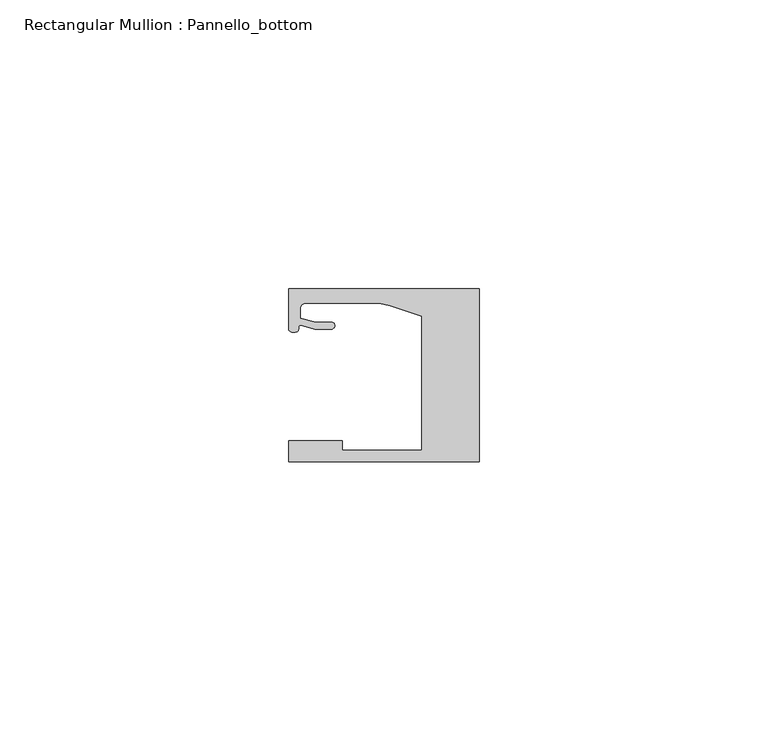
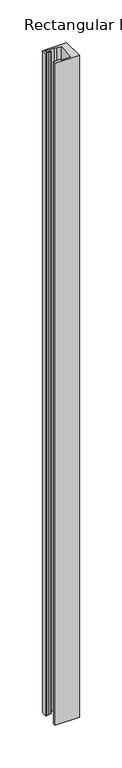
"""IFC4 building model written with IfcOpenShell, lengths in millimetres: member geometry, Rectangular Mullion : Pannello_bottom."""

from ifc_helpers import new_model, si_unit, frame, origin, place, context, project, spatial, polyline, circle_curve, source, transform, mapped, element, save
from ifc_brep_helpers import plane_surface, cylinder_surface, revolved_surface, extruded_surface, spline_curve, advanced_brep


def rectangular_mullion_pannello_bottom_0ebbe626(model_context):
    return source(origin(), model_context, "Body", "AdvancedBrep", [
        advanced_brep(
        [(-33.0, -15.0, 0.0), (0.0, -15.0, 0.0), (0.0, 15.0, 0.0), (-33.0000135, 15.0, 0.0), (-33.0000135, 8.0000472, 0.0), (-30.9223017, 8.6490241, 0.0), (-28.4999305, 7.9999523, 0.0), (-25.59998, 7.9999523, 0.0), (-25.59998, 9.1999523, 0.0), (-28.3419477, 9.1999523, 0.0), (-31.0, 9.9121746, 0.0), (-31.0, 11.4999419, 0.0), (-30.0000002, 12.4999419, 0.0), (-18.5493024, 12.4999438, 0.0), (-15.4591336, 12.0105099, 0.0), (-9.9999723, 10.2367227, 0.0), (-9.9999723, -13.0000004, 0.0), (-23.700041, -13.0000004, 0.0), (-23.700041, -11.3000004, 0.0), (-33.0, -11.3000004, 0.0), (-33.0, -15.0, -950.0), (-33.0, -11.3000004, -950.0), (-23.700041, -11.3000004, -950.0), (-23.700041, -13.0000004, -950.0), (-9.9999723, -13.0000004, -950.0), (-9.9999723, 10.2367227, -950.0), (-15.4591336, 12.0105099, -950.0), (-18.5493024, 12.4999438, -950.0), (-30.0000002, 12.4999419, -950.0), (-31.0, 11.4999419, -950.0), (-31.0, 9.9121746, -950.0), (-28.3419477, 9.1999523, -950.0), (-25.59998, 9.1999523, -950.0), (-25.59998, 7.9999523, -950.0), (-28.4999305, 7.9999523, -950.0), (-30.9223017, 8.6490241, -950.0), (-33.0000135, 8.0000472, -950.0), (-33.0000135, 15.0, -950.0), (0.0, 15.0, -950.0), (0.0, -15.0, -950.0)],
        [
            (0, 1),
            (1, 2),
            (2, 3),
            (3, 4),
            (4, 5, spline_curve(3, [(-33.0000135, 8.0000472, 0.0), (-33.0000135, 7.457047519, 0.0), (-32.262327879, 7.456527435, 0.0), (-31.357433266, 7.563996614, 0.0), (-31.305645054, 7.690065204, 0.0), (-31.298563602, 8.366228555, 0.0), (-31.312054066, 8.717747958, 0.0), (-30.9223017, 8.6490241, 0.0)], [4, 2, 2, 4], [0.0, 0.0027053965905959043, 0.0058611956533709, 0.007702013405570312])),
            (5, 6),
            (6, 7),
            (7, 8, circle_curve(frame((-25.59998, 8.5999523, 0.0), z_axis=(0.0, 0.0, 1.0), x_axis=(0.0, 1.0, 0.0)), 0.6)),
            (8, 9),
            (9, 10),
            (10, 11),
            (11, 12, circle_curve(frame((-30.0, 11.4999419, 0.0), z_axis=(0.0, 0.0, -1.0), x_axis=(0.0, 1.0, 0.0)), 1.0)),
            (12, 13),
            (13, 14, circle_curve(frame((-18.5493007, 2.4999438, 0.0), z_axis=(0.0, 0.0, -1.0), x_axis=(0.0, 1.0, 0.0)), 10.0)),
            (14, 15),
            (15, 16),
            (16, 17),
            (17, 18),
            (18, 19),
            (19, 0),
            (20, 21),
            (21, 22),
            (22, 23),
            (23, 24),
            (24, 25),
            (25, 26),
            (26, 27, circle_curve(frame((-18.5493007, 2.4999438, -950.0), z_axis=(0.0, 0.0, 1.0), x_axis=(0.0, 1.0, 0.0)), 10.0)),
            (27, 28),
            (28, 29, circle_curve(frame((-30.0, 11.4999419, -950.0), z_axis=(0.0, 0.0, 1.0), x_axis=(0.0, 1.0, 0.0)), 1.0)),
            (29, 30),
            (30, 31),
            (31, 32),
            (32, 33, circle_curve(frame((-25.59998, 8.5999523, -950.0), z_axis=(0.0, 0.0, -1.0), x_axis=(0.0, 1.0, 0.0)), 0.6)),
            (33, 34),
            (34, 35),
            (35, 36, spline_curve(3, [(-30.9223017, 8.6490241, -950.0), (-31.312054066, 8.717747958, -950.0), (-31.298563602, 8.366228555, -950.0), (-31.305645054, 7.690065204, -950.0), (-31.357433266, 7.563996614, -950.0), (-32.262327879, 7.456527435, -950.0), (-33.0000135, 7.457047519, -950.0), (-33.0000135, 8.0000472, -950.0)], [4, 2, 2, 4], [0.0, 0.001840817752199412, 0.004996616814974408, 0.007702013405570312])),
            (36, 37),
            (37, 38),
            (38, 39),
            (39, 20),
            (0, 20),
            (39, 1),
            (38, 2),
            (37, 3),
            (36, 4),
            (35, 5),
            (34, 6),
            (33, 7),
            (32, 8),
            (31, 9),
            (30, 10),
            (29, 11),
            (28, 12),
            (27, 13),
            (26, 14),
            (25, 15),
            (24, 16),
            (23, 17),
            (22, 18),
            (21, 19),
        ],
        [
            plane_surface(frame((0.0, -36.2491502, 0.0), z_axis=(0.0, 0.0, 1.0), x_axis=(-1.0, 0.0, 0.0))),
            plane_surface(frame((0.0, -36.2491502, -950.0), z_axis=(0.0, 0.0, -1.0), x_axis=(-1.0, 0.0, 0.0))),
            plane_surface(frame((-33.0, -15.0, 0.0), z_axis=(0.0, -1.0, 0.0), x_axis=(0.0, 0.0, -1.0))),
            plane_surface(frame((0.0, -15.0, 0.0), z_axis=(1.0, 0.0, 0.0), x_axis=(0.0, 0.0, -1.0))),
            plane_surface(frame((0.0, 15.0, 0.0), z_axis=(0.0, 1.0, 0.0), x_axis=(0.0, 0.0, -1.0))),
            plane_surface(frame((-33.0000135, 15.0, 0.0), z_axis=(-1.0, 0.0, 0.0), x_axis=(0.0, 0.0, -1.0))),
            extruded_surface(spline_curve(3, [(-33.0000135, 8.0000472, -950.0), (-33.0000135, 7.457047519, -950.0), (-32.262327879, 7.456527435, -950.0), (-31.357433266, 7.563996614, -950.0), (-31.305645054, 7.690065204, -950.0), (-31.298563602, 8.366228555, -950.0), (-31.312054066, 8.717747958, -950.0), (-30.9223017, 8.6490241, -950.0)], [4, 2, 2, 4], [0.0, 0.0027053965905959043, 0.0058611956533709, 0.007702013405570312]), (0.0, 0.0, 950.0), 950.0),
            plane_surface(frame((-30.9223017, 8.6490241, 0.0), z_axis=(-0.25881883200192934, -0.9659258833891746, 0.0), x_axis=(0.0, 0.0, -1.0))),
            plane_surface(frame((-28.4999305, 7.9999523, 0.0), z_axis=(0.0, -1.0, 0.0), x_axis=(0.0, 0.0, -1.0))),
            cylinder_surface(frame((-25.59998, 8.5999523, 0.0), z_axis=(0.0, 0.0, 1.0), x_axis=(0.0, 1.0, 0.0)), 0.6),
            plane_surface(frame((-25.59998, 9.1999523, 0.0), z_axis=(0.0, 1.0, 0.0), x_axis=(0.0, 0.0, -1.0))),
            plane_surface(frame((-28.3419477, 9.1999523, 0.0), z_axis=(0.25881883204288636, 0.9659258833782002, 0.0), x_axis=(0.0, 0.0, -1.0))),
            plane_surface(frame((-31.0, 9.9121746, 0.0), z_axis=(1.0, 0.0, 0.0), x_axis=(0.0, 0.0, -1.0))),
            revolved_surface(polyline([(-30.0, 12.4999419, -950.0), (-30.0, 12.4999419, 0.0)]), (-30.0, 11.4999419, 0.0), (0.0, 0.0, -1.0)),
            plane_surface(frame((-30.0000002, 12.4999419, 0.0), z_axis=(1.6923026533778639e-07, -0.9999999999999858, 0.0), x_axis=(0.0, 0.0, -1.0))),
            revolved_surface(polyline([(-18.5493007, 12.4999438, -950.0), (-18.5493007, 12.4999438, 0.0)]), (-18.5493007, 2.4999438, 0.0), (0.0, 0.0, -1.0)),
            plane_surface(frame((-15.4591336, 12.0105099, 0.0), z_axis=(-0.30901670911956314, -0.9510566089801992, 0.0), x_axis=(0.0, 0.0, -1.0))),
            plane_surface(frame((-9.9999723, 10.2367227, 0.0), z_axis=(-1.0, 0.0, 0.0), x_axis=(0.0, 0.0, -1.0))),
            plane_surface(frame((-9.9999723, -13.0000004, 0.0), z_axis=(0.0, 1.0, 0.0), x_axis=(0.0, 0.0, -1.0))),
            plane_surface(frame((-23.700041, -13.0000004, 0.0), z_axis=(1.0, 0.0, 0.0), x_axis=(0.0, 0.0, -1.0))),
            plane_surface(frame((-23.700041, -11.3000004, 0.0), z_axis=(0.0, 1.0, 0.0), x_axis=(0.0, 0.0, -1.0))),
            plane_surface(frame((-33.0, -11.3000004, 0.0), z_axis=(-1.0, 0.0, 0.0), x_axis=(0.0, 0.0, -1.0))),
        ],
        [
            (0, [[1, 2, 3, 4, 5, 6, 7, 8, 9, 10, 11, 12, 13, 14, 15, 16, 17, 18, 19, 20]]),
            (1, [[21, 22, 23, 24, 25, 26, 27, 28, 29, 30, 31, 32, 33, 34, 35, 36, 37, 38, 39, 40]]),
            (2, [[-1, 41, -40, 42]]),
            (3, [[-2, -42, -39, 43]]),
            (4, [[-3, -43, -38, 44]]),
            (5, [[-4, -44, -37, 45]]),
            (6, [[-5, -45, -36, 46]]),
            (7, [[-6, -46, -35, 47]]),
            (8, [[-7, -47, -34, 48]]),
            (9, [[-8, -48, -33, 49]]),
            (10, [[-9, -49, -32, 50]]),
            (11, [[-10, -50, -31, 51]]),
            (12, [[-11, -51, -30, 52]]),
            (13, [[-12, -52, -29, 53]]),
            (14, [[-13, -53, -28, 54]]),
            (15, [[-14, -54, -27, 55]]),
            (16, [[-15, -55, -26, 56]]),
            (17, [[-16, -56, -25, 57]]),
            (18, [[-17, -57, -24, 58]]),
            (19, [[-18, -58, -23, 59]]),
            (20, [[-19, -59, -22, 60]]),
            (21, [[-20, -60, -21, -41]]),
        ],
    ),
    ])


if __name__ == "__main__":
    model = new_model("IFC4")
    model_context = context("Model", 3, world=origin())
    ifc_project = project(units=[si_unit("LENGTHUNIT", "METRE", prefix="MILLI")], contexts=[model_context])
    site = spatial("IfcSite", under=ifc_project)
    building = spatial("IfcBuilding", under=site)
    placement = place(None, origin())
    rectangular_mullion_pannello_bottom_shape = rectangular_mullion_pannello_bottom_0ebbe626(model_context)
    element("IfcMember", 1, ObjectType="Rectangular Mullion : Pannello_bottom", at=placement, inside=building, context=model_context, shape_type="MappedRepresentation", body=[
        mapped(rectangular_mullion_pannello_bottom_shape, transform((0.0, 0.0, 0.0), x_axis=(1.0, 0.0, 0.0), y_axis=(0.0, 1.0, 0.0), z_axis=(0.0, 0.0, 1.0))),
    ])
    save(model, "model.ifc")

# Revit data of these elements
# Type "Rectangular Mullion : Pannello_bottom"
#   built-in parameter 1007322 = 0.0984252 (stored number, unit not read)
#   built-in parameter 1007321 = 0.0328083 (stored number, unit not read)
#   built-in parameter 1007320 = 0 (stored number, unit not read)
